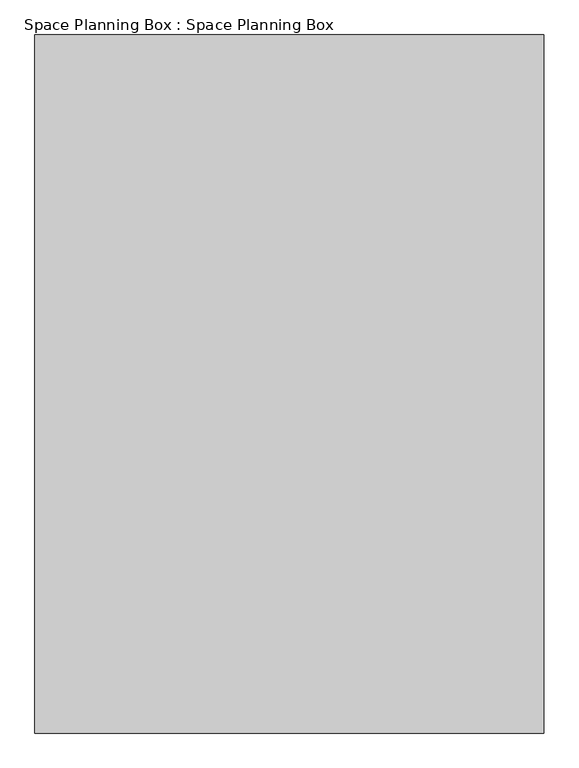
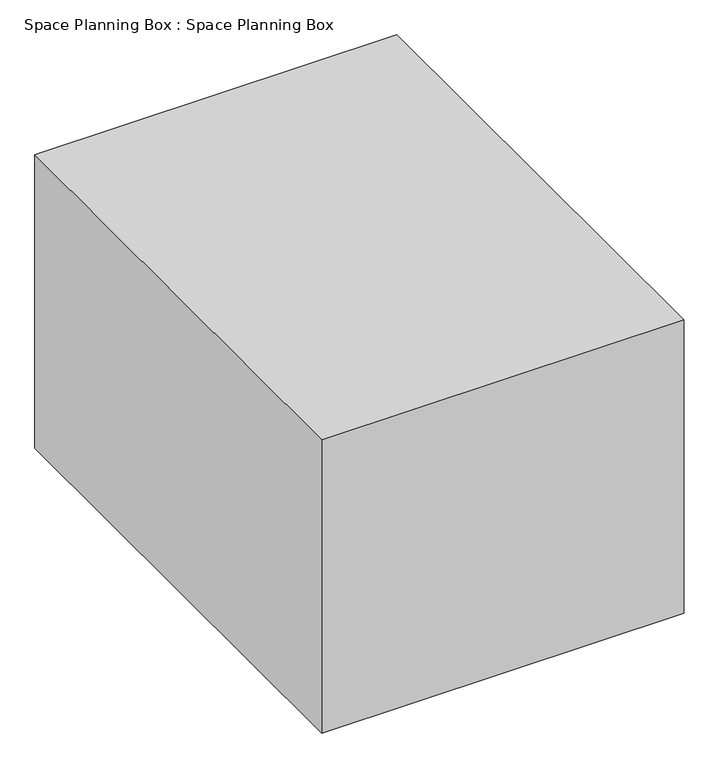
"""IFC4 building model written with IfcOpenShell, lengths in millimetres: proxy geometry, Space Planning Box : Space Planning Box."""

from ifc_helpers import new_model, si_unit, origin, origin_with_axes, place, context, project, spatial, polyline, outline, extrude, source, transform, mapped, element, save


def space_planning_box_space_planning_box_072414e0(model_context):
    return source(origin(), model_context, "Body", "SweptSolid", [
        extrude(outline(polyline([(3500.0, 4800.0), (3500.0, -4800.0), (-3500.0, -4800.0), (-3500.0, 4800.0), (3500.0, 4800.0)])), origin_with_axes(), (0.0, 0.0, 1.0), 6000.0),
    ])


if __name__ == "__main__":
    model = new_model("IFC4")
    model_context = context("Model", 3, world=origin())
    ifc_project = project(units=[si_unit("LENGTHUNIT", "METRE", prefix="MILLI")], contexts=[model_context])
    site = spatial("IfcSite", under=ifc_project)
    building = spatial("IfcBuilding", under=site)
    placement = place(None, origin())
    space_planning_box_space_planning_box_shape = space_planning_box_space_planning_box_072414e0(model_context)
    element("IfcBuildingElementProxy", 1, Name="Space Planning Box : Space Planning Box", ObjectType="Space Planning Box : Space Planning Box", at=placement, inside=building, context=model_context, shape_type="MappedRepresentation", body=[
        mapped(space_planning_box_space_planning_box_shape, transform((0.0, 0.0, 0.0), x_axis=(1.0, 0.0, 0.0), y_axis=(0.0, 1.0, 0.0), z_axis=(0.0, 0.0, 1.0))),
    ])
    save(model, "model.ifc")

# Revit data of these elements
# Type "Space Planning Box : Space Planning Box"
#   Type Comments = "..."
#   Room Name [instance default] = "?"
#   Assembly Code = "..."
#   Width [instance default] = 1524 mm
#   Program Area [instance default] = 0 m²
#   Length [instance default] = 1524 mm
#   Height [instance default] = 1524 mm
#   Area [instance default] = 2.32258 m²
#   Fill Color [instance default] = Cyan
#   Default Elevation = 0
# Element 1 (IfcBuildingElementProxy, "Space Planning Box : Space Planning Box")
#   Room Name = "Kitch & Lunch Room"
#   Width = 7000 mm
#   Program Area = 31.5 m²
#   Length = 9600 mm
#   Height = 6000 mm
#   Area = 67.2 m²
#   Fill Color = Lavender
#   Materials on its faces: "Lavender"
# Materials
#   "Cyan": class "Generic", colour RGB 0 255 255, transparency 0.2, Cost = 0
#   "Lavender": class "Generic", colour RGB 186 85 211, transparency 0.2, Cost = 0
